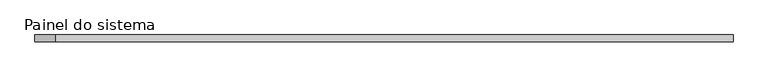
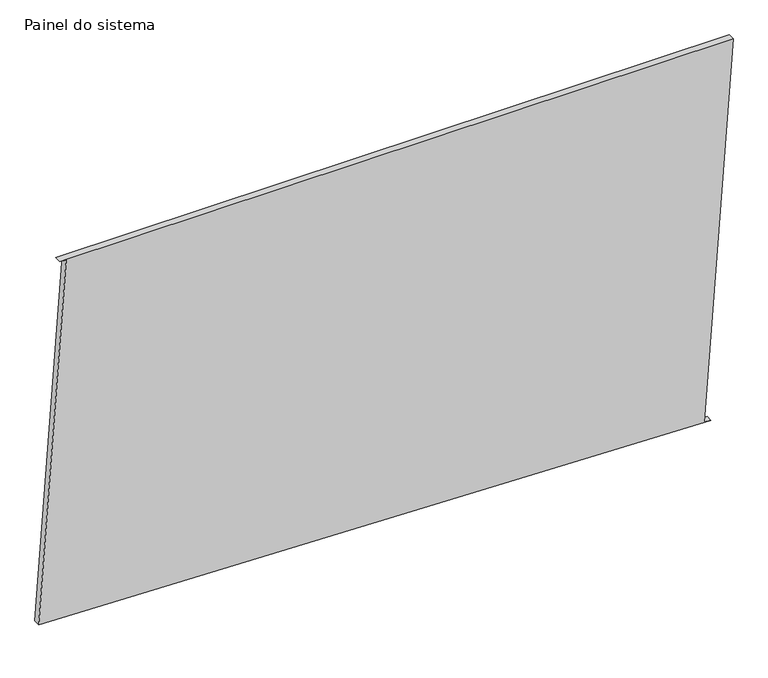
"""IFC4 building model written with IfcOpenShell, lengths in millimetres: plate geometry, Painel do sistema : Envidraçado."""

import ifcopenshell
import ifcopenshell.guid

model = None  # the IFC model being written
_history = None  # IfcOwnerHistory: only IFC2X3 demands one
_inside = {}  # id of a spatial element -> (the spatial element, [elements in it])
_under = {}  # id of a project, library or spatial element -> (it, [spatial elements below it])
_declared = {}  # id of a project -> (the project, [libraries it declares])
_typed = {}  # id of a type object -> (the type object, [elements of that type])
_made_of = {}  # id of a material, layer set ... -> (it, [elements and type objects made of it])


def new_model(schema):
    """Start an empty IFC model of exactly this schema.

    Asked for "IFC4X3", IfcOpenShell would pick the latest addendum, in which some entities
    have other attributes; the version numbers below select the first issue.
    IFC2X3 requires an IfcOwnerHistory on every rooted entity: one is made here for all.
    """
    global model, _history
    if schema == "IFC4X3":
        model = ifcopenshell.file(schema_version=(4, 3, 0, 0))
    else:
        model = ifcopenshell.file(schema=schema)
    _inside.clear()
    _under.clear()
    _declared.clear()
    _typed.clear()
    _made_of.clear()
    _history = None
    if model.schema == "IFC2X3":
        org = make("IfcOrganization", Name="unknown")
        user = make(
            "IfcPersonAndOrganization",
            ThePerson=make("IfcPerson", FamilyName="unknown"),
            TheOrganization=org,
        )
        app = make(
            "IfcApplication",
            ApplicationDeveloper=org,
            Version="unknown",
            ApplicationFullName="unknown",
            ApplicationIdentifier="unknown",
        )
        _history = make(
            "IfcOwnerHistory",
            OwningUser=user,
            OwningApplication=app,
            ChangeAction="ADDED",
            CreationDate=0,
        )
    return model


def make(cls, **values):
    """One entity of the class cls with the attributes given. An attribute that is None is left unset."""
    return model.create_entity(
        cls, **{name: value for name, value in values.items() if value is not None}
    )


def rooted(cls, **values):
    """An entity with a GlobalId (a new one), such as an element, a storey or a relation."""
    return make(cls, GlobalId=ifcopenshell.guid.new(), OwnerHistory=_history, **values)


def si_unit(unit_type, name, prefix=None):
    """IfcSIUnit, for example si_unit("LENGTHUNIT", "METRE", prefix="MILLI")."""
    return make("IfcSIUnit", UnitType=unit_type, Prefix=prefix, Name=name)


def assignment(units):
    """IfcUnitAssignment: the units of a project."""
    return None if units is None else make("IfcUnitAssignment", Units=units)


def point(xyz):
    """IfcCartesianPoint."""
    return None if xyz is None else make("IfcCartesianPoint", Coordinates=xyz)


def direction(xyz):
    """IfcDirection."""
    return None if xyz is None else make("IfcDirection", DirectionRatios=xyz)


def frame(location, z_axis=None, x_axis=None):
    """IfcAxis2Placement3D, a coordinate frame: its origin and axes. An axis left out is left unset."""
    return make(
        "IfcAxis2Placement3D",
        Location=point(location),
        Axis=direction(z_axis),
        RefDirection=direction(x_axis),
    )


def origin():
    """The frame at (0, 0, 0) with its axes left unset."""
    return frame((0.0, 0.0, 0.0))


def place(relative_to, where):
    """IfcLocalPlacement: puts the frame where relative to a parent placement (None: the world)."""
    return make(
        "IfcLocalPlacement", PlacementRelTo=relative_to, RelativePlacement=where
    )


def context(
    kind, dimensions, precision=None, world=None, true_north=None, identifier=None
):
    """IfcGeometricRepresentationContext, for example the 3D "Model" context."""
    return make(
        "IfcGeometricRepresentationContext",
        ContextIdentifier=identifier,
        ContextType=kind,
        CoordinateSpaceDimension=dimensions,
        Precision=precision,
        WorldCoordinateSystem=world,
        TrueNorth=true_north,
    )


def project(units=None, contexts=None):
    """IfcProject with its units and contexts."""
    return rooted(
        "IfcProject",
        Name="project",
        RepresentationContexts=contexts,
        UnitsInContext=assignment(units),
    )


def spatial(cls, under=None, at=None, **own):
    """A site, building, storey or space (cls), placed at a placement, below another one or the project."""
    s = rooted(cls, ObjectPlacement=at, **own)
    if under is not None:
        _under.setdefault(under.id(), (under, []))[1].append(s)
    return s


def polyline(points):
    """IfcPolyline through the points."""
    return make("IfcPolyline", Points=[point(p) for p in points])


def outline(outer, holes=None, kind="AREA"):
    """IfcArbitraryClosedProfileDef: a profile drawn as a closed curve; with holes, ...WithVoids."""
    if holes is None:
        return make("IfcArbitraryClosedProfileDef", ProfileType=kind, OuterCurve=outer)
    return make(
        "IfcArbitraryProfileDefWithVoids",
        ProfileType=kind,
        OuterCurve=outer,
        InnerCurves=holes,
    )


def extrude(swept, where, along, depth):
    """IfcExtrudedAreaSolid: the profile swept, set in the frame where, extruded along a direction by depth."""
    return make(
        "IfcExtrudedAreaSolid",
        SweptArea=swept,
        Position=where,
        ExtrudedDirection=direction(along),
        Depth=depth,
    )


def shape(context_of_items, identifier, shape_type, items):
    """IfcShapeRepresentation: the items that make up one representation, for example the "Body"."""
    return make(
        "IfcShapeRepresentation",
        ContextOfItems=context_of_items,
        RepresentationIdentifier=identifier,
        RepresentationType=shape_type,
        Items=items,
    )


def source(mapping_origin, context_of_items, identifier, shape_type, items):
    """IfcRepresentationMap: a shape defined once, which mapped items show again and again."""
    return make(
        "IfcRepresentationMap",
        MappingOrigin=mapping_origin,
        MappedRepresentation=shape(context_of_items, identifier, shape_type, items),
    )


def transform(
    local_origin,
    x_axis=None,
    y_axis=None,
    z_axis=None,
    scale=None,
    scale2=None,
    scale3=None,
    uniform=True,
):
    """IfcCartesianTransformationOperator3D, or its non-uniform kind. x_axis, y_axis, z_axis: its Axis1, 2, 3."""
    if uniform:
        return make(
            "IfcCartesianTransformationOperator3D",
            Axis1=direction(x_axis),
            Axis2=direction(y_axis),
            LocalOrigin=point(local_origin),
            Scale=scale,
            Axis3=direction(z_axis),
        )
    return make(
        "IfcCartesianTransformationOperator3DnonUniform",
        Axis1=direction(x_axis),
        Axis2=direction(y_axis),
        LocalOrigin=point(local_origin),
        Scale=scale,
        Axis3=direction(z_axis),
        Scale2=scale2,
        Scale3=scale3,
    )


def mapped(mapping_source, mapping_target):
    """IfcMappedItem: shows the shape of a source again, moved by a transform."""
    return make(
        "IfcMappedItem", MappingSource=mapping_source, MappingTarget=mapping_target
    )


def made_of(thing, what):
    """Note that an element or type object is made of a material, layer set ...; save() writes the relation."""
    if what is not None:
        _made_of.setdefault(what.id(), (what, []))[1].append(thing)
    return thing


def element(
    cls,
    number,
    at=None,
    inside=None,
    cuts=None,
    type_object=None,
    material=None,
    context=None,
    identifier="Body",
    shape_type=None,
    held_by="IfcProductDefinitionShape",
    body=None,
    shapes=None,
    **own,
):
    """One element of the class cls, such as IfcWall. Its Tag is "e" and its number.

    at: its placement. inside: the storey or other place that contains it. cuts: it is an
    opening in that element (IfcRelVoidsElement). A single representation is given by context,
    identifier, shape_type and body (its items); several are given by shapes. held_by: the class
    of the entity that holds the representations. save() writes the other relations.
    """
    e = rooted(cls, Tag="e%d" % number, ObjectPlacement=at, **own)
    if body is not None:
        shapes = [shape(context, identifier, shape_type, body)]
    if shapes is not None:
        e.Representation = make(held_by, Representations=shapes)
    if inside is not None:
        _inside.setdefault(inside.id(), (inside, []))[1].append(e)
    if cuts is not None:
        rooted(
            "IfcRelVoidsElement", RelatingBuildingElement=cuts, RelatedOpeningElement=e
        )
    if type_object is not None:
        _typed.setdefault(type_object.id(), (type_object, []))[1].append(e)
    return made_of(e, material)


def aggregate(whole, parts):
    """IfcRelAggregates: a whole, such as a stair, and the parts it consists of."""
    return rooted("IfcRelAggregates", RelatingObject=whole, RelatedObjects=parts)


def save(model, path):
    """Write the relations noted so far, then the file.

    IfcRelAggregates (storeys below a building ...), IfcRelContainedInSpatialStructure (elements
    in a storey), IfcRelDefinesByType, IfcRelAssociatesMaterial and IfcRelDeclares: one each for
    every whole, place, type object, material and project.
    """
    for whole, parts in _under.values():
        aggregate(whole, parts)
    for where, things in _inside.values():
        rooted(
            "IfcRelContainedInSpatialStructure",
            RelatedElements=things,
            RelatingStructure=where,
        )
    for kind, things in _typed.values():
        rooted("IfcRelDefinesByType", RelatedObjects=things, RelatingType=kind)
    for what, things in _made_of.values():
        rooted("IfcRelAssociatesMaterial", RelatedObjects=things, RelatingMaterial=what)
    for by, libraries in _declared.values():
        rooted("IfcRelDeclares", RelatingContext=by, RelatedDefinitions=libraries)
    model.write(path)


def painel_do_sistema_41d4a81c(model_context):
    return source(origin(), model_context, "Body", "SweptSolid", [
        extrude(outline(polyline([(0.0, 1232.3407402), (1.8159485, 1207.4067808), (1502.3167726, 1316.6887507), (1502.3167726, -1237.6878906), (1500.5008241, -1212.7539312), (73.4192812, -1316.6887507), (0.0, 1232.3407402)])), frame((0.0, 24.5, 0.0), z_axis=(0.0, 1.0, 0.0), x_axis=(0.0, 0.0, 1.0)), (0.0, 0.0, 1.0), 25.0),
    ])


if __name__ == "__main__":
    model = new_model("IFC4")
    model_context = context("Model", 3, world=origin())
    ifc_project = project(units=[si_unit("LENGTHUNIT", "METRE", prefix="MILLI")], contexts=[model_context])
    site = spatial("IfcSite", under=ifc_project)
    building = spatial("IfcBuilding", under=site)
    placement = place(None, origin())
    painel_do_sistema_shape = painel_do_sistema_41d4a81c(model_context)
    element("IfcPlate", 1, ObjectType="Painel do sistema : Envidraçado", at=placement, inside=building, context=model_context, shape_type="MappedRepresentation", body=[
        mapped(painel_do_sistema_shape, transform((0.0, 0.0, 0.0), x_axis=(1.0, 0.0, 0.0), y_axis=(0.0, 1.0, 0.0), z_axis=(0.0, 0.0, 1.0))),
    ])
    save(model, "model.ifc")

# Revit data of these elements
# Type "Painel do sistema : Envidraçado"
#   Construction Type Id = "GSP4R"
#   Analytic Construction = "Vidraça única Pilkington 1/8 pol"
#   Visual Light Transmittance = 0.9
#   Solar Heat Gain Coefficient = 0.86
#   Heat Transfer Coefficient (U) = 6.7069 W/(m²·K)
# Element 1 (IfcPlate, "Painel do sistema : Envidraçado")
#   Materials on its faces: "Vidro"
# Materials
#   "Vidro": class "Vidro", colour RGB 0 128 192, transparency 0.9, Description = "Vidro de sílica", Cost = 0
